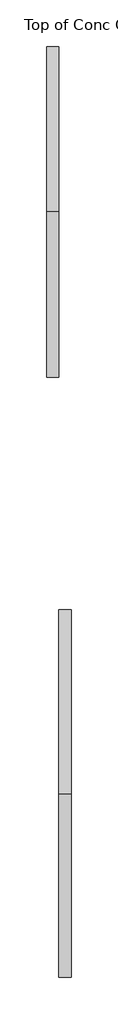
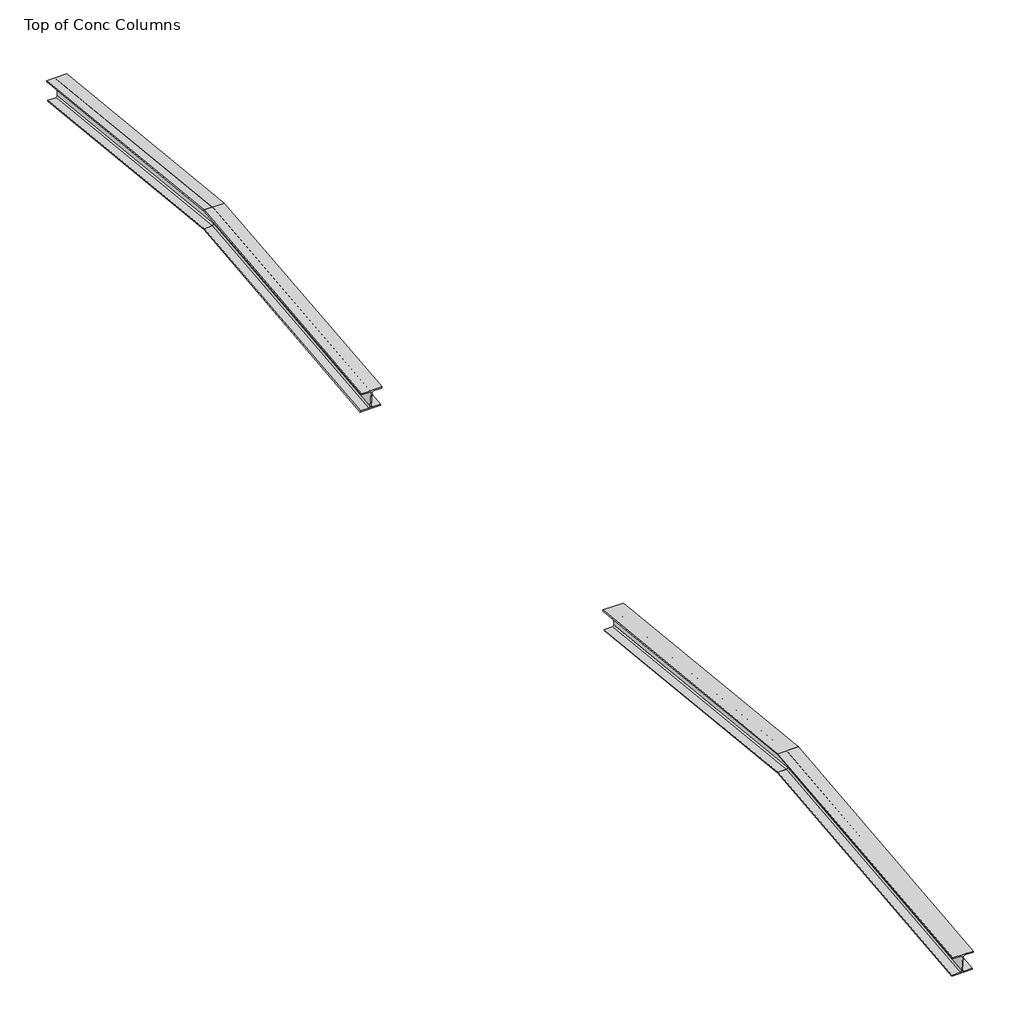
# One storey: 4 beams.
"""IFC4 building model written with IfcOpenShell, lengths in millimetres."""

from ifc_helpers import new_model, si_unit, frame, origin, place, context, project, spatial, polyline, circle_curve, ellipse_curve, element, save
from ifc_brep_helpers import plane_surface, revolved_surface, advanced_brep

model = new_model("IFC4")

# Units and contexts
model_context = context("Model", 3, world=origin())
ifc_project = project(units=[si_unit("LENGTHUNIT", "METRE", prefix="MILLI")], contexts=[model_context])

# Site, building, storey
site = spatial("IfcSite", under=ifc_project)
building = spatial("IfcBuilding", under=site)
storey = spatial("IfcBuildingStorey", under=building, Name="Top of Conc Columns", Elevation=33782.0)

# Beams
placement = place(None, origin())
element("IfcBeam", 1, ObjectType="W-Wide Flange : W12X79", at=placement, inside=storey, context=model_context, shape_type="AdvancedBrep", body=[
    advanced_brep(
    [(-21755.4154607, 20969.2190095, 33178.8039345), (-21630.3204607, 20969.2190095, 33178.8039345), (-21607.7144607, 20971.5967656, 33201.2845375), (-21607.7144607, 20996.0422355, 33432.4053438), (-21630.3204607, 20998.4199915, 33454.8859468), (-21755.4154607, 20998.4199915, 33454.8859468), (-21755.4154607, 21000.383644, 33473.4513887), (-21448.0754607, 21000.383644, 33473.4513887), (-21448.0754607, 20998.4199915, 33454.8859468), (-21573.1704607, 20998.4199915, 33454.8859468), (-21595.7764607, 20996.0422355, 33432.4053438), (-21595.7764607, 20971.5967656, 33201.2845375), (-21573.1704607, 20969.2190095, 33178.8039345), (-21448.0754607, 20969.2190095, 33178.8039345), (-21448.0754607, 20967.255357, 33160.2384927), (-21755.4154607, 20967.255357, 33160.2384927), (-21755.4154607, 16882.4695005, 33611.0562864), (-21630.3204607, 16882.4695005, 33611.0562864), (-21607.7144607, 16882.4695005, 33633.7883829), (-21607.7144607, 16882.4695005, 33867.4947677), (-21630.3204607, 16882.4695005, 33890.2268642), (-21755.4154607, 16882.4695005, 33890.2268642), (-21755.4154607, 16882.4695005, 33909.0), (-21448.0754607, 16882.4695005, 33909.0), (-21448.0754607, 16882.4695005, 33890.2268642), (-21573.1704607, 16882.4695005, 33890.2268642), (-21595.7764607, 16882.4695005, 33867.4947677), (-21595.7764607, 16882.4695005, 33633.7883829), (-21573.1704607, 16882.4695005, 33611.0562864), (-21448.0754607, 16882.4695005, 33611.0562864), (-21448.0754607, 16882.4695005, 33592.2831506), (-21755.4154607, 16882.4695005, 33592.2831506)],
    [
        (0, 1),
        (1, 2, circle_curve(frame((-21630.3204607, 20971.5967656, 33201.2845375), z_axis=(0.0, -0.9944529335787645, 0.10518252182083104), x_axis=(1.0, 0.0, 0.0)), 22.606)),
        (2, 3),
        (3, 4, circle_curve(frame((-21630.3204607, 20996.0422355, 33432.4053438), z_axis=(0.0, -0.9944529335787645, 0.10518252182083104), x_axis=(1.0, 0.0, 0.0)), 22.606)),
        (4, 5),
        (5, 6),
        (6, 7),
        (7, 8),
        (8, 9),
        (9, 10, circle_curve(frame((-21573.1704607, 20996.0422355, 33432.4053438), z_axis=(0.0, -0.9944529335787645, 0.10518252182083104), x_axis=(1.0, 0.0, 0.0)), 22.606)),
        (10, 11),
        (11, 12, circle_curve(frame((-21573.1704607, 20971.5967656, 33201.2845375), z_axis=(0.0, -0.9944529335787645, 0.10518252182083104), x_axis=(1.0, 0.0, 0.0)), 22.606)),
        (12, 13),
        (13, 14),
        (14, 15),
        (15, 0),
        (0, 16),
        (16, 17),
        (17, 1),
        (17, 18, ellipse_curve(frame((-21630.3204607, 16882.4695005, 33633.7883829), z_axis=(0.0, -1.0, 0.0), x_axis=(0.0, 0.0, 0.9999999999999999)), 22.7320964, 22.606)),
        (18, 2),
        (18, 19),
        (19, 3),
        (19, 20, ellipse_curve(frame((-21630.3204607, 16882.4695005, 33867.4947677), z_axis=(0.0, -1.0, 0.0), x_axis=(0.0, 0.0, 0.9999999999999999)), 22.7320964, 22.606)),
        (20, 4),
        (20, 21),
        (21, 5),
        (21, 22),
        (22, 6),
        (22, 23),
        (23, 7),
        (23, 24),
        (24, 8),
        (24, 25),
        (25, 9),
        (25, 26, ellipse_curve(frame((-21573.1704607, 16882.4695005, 33867.4947677), z_axis=(0.0, -1.0, 0.0), x_axis=(0.0, 0.0, 0.9999999999999999)), 22.7320964, 22.606)),
        (26, 10),
        (26, 27),
        (27, 11),
        (27, 28, ellipse_curve(frame((-21573.1704607, 16882.4695005, 33633.7883829), z_axis=(0.0, -1.0, 0.0), x_axis=(0.0, 0.0, 0.9999999999999999)), 22.7320964, 22.606)),
        (28, 12),
        (28, 29),
        (29, 13),
        (29, 30),
        (30, 14),
        (30, 31),
        (31, 15),
        (31, 16),
    ],
    [
        plane_surface(frame((-21601.7454607, 20983.8195005, 33316.8449407), z_axis=(0.0, 0.9944529335787644, -0.10518252182083183), x_axis=(0.0, 0.10518252182083183, 0.9944529335787644))),
        plane_surface(frame((-21755.4154607, 20969.2190095, 33178.8039345), z_axis=(0.0, 0.10518252182083103, 0.9944529335787644), x_axis=(0.0, -0.9944529335787644, 0.10518252182083103))),
        revolved_surface(polyline([(-21607.7144607, 16880.091744411304, 33634.03987627958), (-21607.7144607, 20971.5967656, 33201.2845375)]), (-21630.3204607, 20971.5967656, 33201.2845375), (0.0, -0.9944529335787643, 0.10518252182083102)),
        plane_surface(frame((-21607.7144607, 20971.5967656, 33201.2845375), z_axis=(-1.0, 0.0, 0.0), x_axis=(0.0, -0.9944529335787644, 0.10518252182083103))),
        revolved_surface(polyline([(-21607.7144607, 16880.09174440577, 33867.74626112727), (-21607.7144607, 20996.0422355, 33432.4053438)]), (-21630.3204607, 20996.0422355, 33432.4053438), (0.0, -0.9944529335787643, 0.10518252182083102)),
        plane_surface(frame((-21630.3204607, 20998.4199915, 33454.8859468), z_axis=(0.0, -0.10518252182083103, -0.9944529335787644), x_axis=(0.0, -0.9944529335787644, 0.10518252182083103))),
        plane_surface(frame((-21755.4154607, 20998.4199915, 33454.8859468), z_axis=(-1.0, 0.0, 0.0), x_axis=(0.0, -0.9944529335787644, 0.10518252182083103))),
        plane_surface(frame((-21755.4154607, 21000.383644, 33473.4513887), z_axis=(0.0, 0.10518252182083103, 0.9944529335787644), x_axis=(0.0, -0.9944529335787644, 0.10518252182083103))),
        plane_surface(frame((-21448.0754607, 21000.383644, 33473.4513887), z_axis=(1.0, 0.0, 0.0), x_axis=(0.0, -0.9944529335787644, 0.10518252182083103))),
        plane_surface(frame((-21448.0754607, 20998.4199915, 33454.8859468), z_axis=(0.0, -0.10518252182083103, -0.9944529335787644), x_axis=(0.0, -0.9944529335787644, 0.10518252182083103))),
        revolved_surface(polyline([(-21550.5644607, 16880.09174440577, 33867.74626112727), (-21550.5644607, 20996.0422355, 33432.4053438)]), (-21573.1704607, 20996.0422355, 33432.4053438), (0.0, -0.9944529335787643, 0.10518252182083102)),
        plane_surface(frame((-21595.7764607, 20996.0422355, 33432.4053438), z_axis=(1.0, 0.0, 0.0), x_axis=(0.0, -0.9944529335787644, 0.10518252182083103))),
        revolved_surface(polyline([(-21550.5644607, 16880.091744411304, 33634.03987627958), (-21550.5644607, 20971.5967656, 33201.2845375)]), (-21573.1704607, 20971.5967656, 33201.2845375), (0.0, -0.9944529335787643, 0.10518252182083102)),
        plane_surface(frame((-21573.1704607, 20969.2190095, 33178.8039345), z_axis=(0.0, 0.10518252182083103, 0.9944529335787644), x_axis=(0.0, -0.9944529335787644, 0.10518252182083103))),
        plane_surface(frame((-21448.0754607, 20969.2190095, 33178.8039345), z_axis=(1.0, 0.0, 0.0), x_axis=(0.0, -0.9944529335787644, 0.10518252182083103))),
        plane_surface(frame((-21448.0754607, 20967.255357, 33160.2384927), z_axis=(0.0, -0.10518252182083103, -0.9944529335787644), x_axis=(0.0, -0.9944529335787644, 0.10518252182083103))),
        plane_surface(frame((-21755.4154607, 20967.255357, 33160.2384927), z_axis=(-1.0, 0.0, 0.0), x_axis=(0.0, -0.9944529335787644, 0.10518252182083103))),
        plane_surface(frame((-21601.7454607, 16882.4695005, 33592.2831506), z_axis=(0.0, -1.0, 0.0), x_axis=(0.0, 0.0, 1.0))),
    ],
    [
        (0, [[1, 2, 3, 4, 5, 6, 7, 8, 9, 10, 11, 12, 13, 14, 15, 16]]),
        (1, [[-1, 17, 18, 19]]),
        (2, [[-2, -19, 20, 21]]),
        (3, [[-3, -21, 22, 23]]),
        (4, [[-4, -23, 24, 25]]),
        (5, [[-5, -25, 26, 27]]),
        (6, [[-6, -27, 28, 29]]),
        (7, [[-7, -29, 30, 31]]),
        (8, [[-8, -31, 32, 33]]),
        (9, [[-9, -33, 34, 35]]),
        (10, [[-10, -35, 36, 37]]),
        (11, [[-11, -37, 38, 39]]),
        (12, [[-12, -39, 40, 41]]),
        (13, [[-13, -41, 42, 43]]),
        (14, [[-14, -43, 44, 45]]),
        (15, [[-15, -45, 46, 47]]),
        (16, [[-16, -47, 48, -17]]),
        (17, [[-48, -46, -44, -42, -40, -38, -36, -34, -32, -30, -28, -26, -24, -22, -20, -18]]),
    ],
),
])
element("IfcBeam", 2, ObjectType="W-Wide Flange : W12X79", at=placement, inside=storey, context=model_context, shape_type="AdvancedBrep", body=[
    advanced_brep(
    [(-21755.4154607, 12795.7199915, 33178.8039345), (-21755.4154607, 12797.683644, 33160.2384927), (-21448.0754607, 12797.683644, 33160.2384927), (-21448.0754607, 12795.7199915, 33178.8039345), (-21573.1704607, 12795.7199915, 33178.8039345), (-21595.7764607, 12793.3422355, 33201.2845375), (-21595.7764607, 12768.8967656, 33432.4053438), (-21573.1704607, 12766.5190095, 33454.8859468), (-21448.0754607, 12766.5190095, 33454.8859468), (-21448.0754607, 12764.555357, 33473.4513887), (-21755.4154607, 12764.555357, 33473.4513887), (-21755.4154607, 12766.5190095, 33454.8859468), (-21630.3204607, 12766.5190095, 33454.8859468), (-21607.7144607, 12768.8967656, 33432.4053438), (-21607.7144607, 12793.3422355, 33201.2845375), (-21630.3204607, 12795.7199915, 33178.8039345), (-21630.3204607, 16882.4695005, 33611.0562864), (-21755.4154607, 16882.4695005, 33611.0562864), (-21607.7144607, 16882.4695005, 33633.7883829), (-21607.7144607, 16882.4695005, 33867.4947677), (-21630.3204607, 16882.4695005, 33890.2268642), (-21755.4154607, 16882.4695005, 33890.2268642), (-21755.4154607, 16882.4695005, 33909.0), (-21448.0754607, 16882.4695005, 33909.0), (-21448.0754607, 16882.4695005, 33890.2268642), (-21573.1704607, 16882.4695005, 33890.2268642), (-21595.7764607, 16882.4695005, 33867.4947677), (-21595.7764607, 16882.4695005, 33633.7883829), (-21573.1704607, 16882.4695005, 33611.0562864), (-21448.0754607, 16882.4695005, 33611.0562864), (-21448.0754607, 16882.4695005, 33592.2831506), (-21755.4154607, 16882.4695005, 33592.2831506)],
    [
        (0, 1),
        (1, 2),
        (2, 3),
        (3, 4),
        (4, 5, circle_curve(frame((-21573.1704607, 12793.3422355, 33201.2845375), z_axis=(0.0, 0.9944529335787644, 0.10518252182083103), x_axis=(1.0, 0.0, 0.0)), 22.606)),
        (5, 6),
        (6, 7, circle_curve(frame((-21573.1704607, 12768.8967656, 33432.4053438), z_axis=(0.0, 0.9944529335787644, 0.10518252182083103), x_axis=(1.0, 0.0, 0.0)), 22.606)),
        (7, 8),
        (8, 9),
        (9, 10),
        (10, 11),
        (11, 12),
        (12, 13, circle_curve(frame((-21630.3204607, 12768.8967656, 33432.4053438), z_axis=(0.0, 0.9944529335787644, 0.10518252182083103), x_axis=(1.0, 0.0, 0.0)), 22.606)),
        (13, 14),
        (14, 15, circle_curve(frame((-21630.3204607, 12793.3422355, 33201.2845375), z_axis=(0.0, 0.9944529335787644, 0.10518252182083103), x_axis=(1.0, 0.0, 0.0)), 22.606)),
        (15, 0),
        (15, 16),
        (16, 17),
        (17, 0),
        (14, 18),
        (18, 16, ellipse_curve(frame((-21630.3204607, 16882.4695005, 33633.7883829), z_axis=(0.0, 1.0, 0.0), x_axis=(0.0, 0.0, 1.0)), 22.7320964, 22.606)),
        (13, 19),
        (19, 18),
        (12, 20),
        (20, 19, ellipse_curve(frame((-21630.3204607, 16882.4695005, 33867.4947677), z_axis=(0.0, 1.0, 0.0), x_axis=(0.0, 0.0, 1.0)), 22.7320964, 22.606)),
        (11, 21),
        (21, 20),
        (10, 22),
        (22, 21),
        (9, 23),
        (23, 22),
        (8, 24),
        (24, 23),
        (7, 25),
        (25, 24),
        (6, 26),
        (26, 25, ellipse_curve(frame((-21573.1704607, 16882.4695005, 33867.4947677), z_axis=(0.0, 1.0, 0.0), x_axis=(0.0, 0.0, 1.0)), 22.7320964, 22.606)),
        (5, 27),
        (27, 26),
        (4, 28),
        (28, 27, ellipse_curve(frame((-21573.1704607, 16882.4695005, 33633.7883829), z_axis=(0.0, 1.0, 0.0), x_axis=(0.0, 0.0, 1.0)), 22.7320964, 22.606)),
        (3, 29),
        (29, 28),
        (2, 30),
        (30, 29),
        (1, 31),
        (31, 30),
        (17, 31),
    ],
    [
        plane_surface(frame((-21601.7454607, 12781.1195005, 33316.8449407), z_axis=(0.0, -0.9944529335787644, -0.10518252182083185), x_axis=(0.0, -0.10518252182083185, 0.9944529335787644))),
        plane_surface(frame((-21755.4154607, 12795.7199915, 33178.8039345), z_axis=(0.0, -0.10518252182083103, 0.9944529335787644), x_axis=(0.0, 0.9944529335787644, 0.10518252182083103))),
        revolved_surface(polyline([(-21607.7144607, 16884.847256589805, 33634.03987626912), (-21607.7144607, 12793.342235414419, 33201.28453749095)]), (-21630.3204607, 12793.3422355, 33201.2845375), (0.0, 0.9944529335787644, 0.10518252182083103)),
        plane_surface(frame((-21607.7144607, 12793.3422355, 33201.2845375), z_axis=(-1.0, 0.0, 0.0), x_axis=(0.0, 0.9944529335787644, 0.10518252182083103))),
        revolved_surface(polyline([(-21607.7144607, 16884.847256595338, 33867.746261116816), (-21607.7144607, 12768.896765586687, 33432.405343798586)]), (-21630.3204607, 12768.8967656, 33432.4053438), (0.0, 0.9944529335787644, 0.10518252182083103)),
        plane_surface(frame((-21630.3204607, 12766.5190095, 33454.8859468), z_axis=(0.0, 0.10518252182083103, -0.9944529335787644), x_axis=(0.0, 0.9944529335787644, 0.10518252182083103))),
        plane_surface(frame((-21755.4154607, 12766.5190095, 33454.8859468), z_axis=(-1.0, 0.0, 0.0), x_axis=(0.0, 0.9944529335787644, 0.10518252182083103))),
        plane_surface(frame((-21755.4154607, 12764.555357, 33473.4513887), z_axis=(0.0, -0.10518252182083103, 0.9944529335787644), x_axis=(0.0, 0.9944529335787644, 0.10518252182083103))),
        plane_surface(frame((-21448.0754607, 12764.555357, 33473.4513887), z_axis=(1.0, 0.0, 0.0), x_axis=(0.0, 0.9944529335787644, 0.10518252182083103))),
        plane_surface(frame((-21448.0754607, 12766.5190095, 33454.8859468), z_axis=(0.0, 0.10518252182083103, -0.9944529335787644), x_axis=(0.0, 0.9944529335787644, 0.10518252182083103))),
        revolved_surface(polyline([(-21550.5644607, 16884.847256595338, 33867.746261116816), (-21550.5644607, 12768.896765586687, 33432.405343798586)]), (-21573.1704607, 12768.8967656, 33432.4053438), (0.0, 0.9944529335787644, 0.10518252182083103)),
        plane_surface(frame((-21595.7764607, 12768.8967656, 33432.4053438), z_axis=(1.0, 0.0, 0.0), x_axis=(0.0, 0.9944529335787644, 0.10518252182083103))),
        revolved_surface(polyline([(-21550.5644607, 16884.847256589805, 33634.03987626912), (-21550.5644607, 12793.342235414419, 33201.28453749095)]), (-21573.1704607, 12793.3422355, 33201.2845375), (0.0, 0.9944529335787644, 0.10518252182083103)),
        plane_surface(frame((-21573.1704607, 12795.7199915, 33178.8039345), z_axis=(0.0, -0.10518252182083103, 0.9944529335787644), x_axis=(0.0, 0.9944529335787644, 0.10518252182083103))),
        plane_surface(frame((-21448.0754607, 12795.7199915, 33178.8039345), z_axis=(1.0, 0.0, 0.0), x_axis=(0.0, 0.9944529335787644, 0.10518252182083103))),
        plane_surface(frame((-21448.0754607, 12797.683644, 33160.2384927), z_axis=(0.0, 0.10518252182083103, -0.9944529335787644), x_axis=(0.0, 0.9944529335787644, 0.10518252182083103))),
        plane_surface(frame((-21755.4154607, 12797.683644, 33160.2384927), z_axis=(-1.0, 0.0, 0.0), x_axis=(0.0, 0.9944529335787644, 0.10518252182083103))),
        plane_surface(frame((-21601.7454607, 16882.4695005, 33592.2831506), z_axis=(0.0, 1.0, 0.0), x_axis=(0.0, 0.0, -1.0))),
    ],
    [
        (0, [[1, 2, 3, 4, 5, 6, 7, 8, 9, 10, 11, 12, 13, 14, 15, 16]]),
        (1, [[17, 18, 19, -16]]),
        (2, [[20, 21, -17, -15]]),
        (3, [[22, 23, -20, -14]]),
        (4, [[24, 25, -22, -13]]),
        (5, [[26, 27, -24, -12]]),
        (6, [[28, 29, -26, -11]]),
        (7, [[30, 31, -28, -10]]),
        (8, [[32, 33, -30, -9]]),
        (9, [[34, 35, -32, -8]]),
        (10, [[36, 37, -34, -7]]),
        (11, [[38, 39, -36, -6]]),
        (12, [[40, 41, -38, -5]]),
        (13, [[42, 43, -40, -4]]),
        (14, [[44, 45, -42, -3]]),
        (15, [[46, 47, -44, -2]]),
        (16, [[-19, 48, -46, -1]]),
        (17, [[-18, -21, -23, -25, -27, -29, -31, -33, -35, -37, -39, -41, -43, -45, -47, -48]]),
    ],
),
])
element("IfcBeam", 3, ObjectType="W-Wide Flange : W12X79", at=placement, inside=storey, context=model_context, shape_type="AdvancedBrep", body=[
    advanced_brep(
    [(-21450.6154607, 6948.4190095, 33130.4462422), (-21325.5204607, 6948.4190095, 33130.4462422), (-21302.9144607, 6950.7967656, 33152.9268452), (-21302.9144607, 6975.2422355, 33384.0476515), (-21325.5204607, 6977.6199915, 33406.5282545), (-21450.6154607, 6977.6199915, 33406.5282545), (-21450.6154607, 6979.583644, 33425.0936964), (-21143.2754607, 6979.583644, 33425.0936964), (-21143.2754607, 6977.6199915, 33406.5282545), (-21268.3704607, 6977.6199915, 33406.5282545), (-21290.9764607, 6975.2422355, 33384.0476515), (-21290.9764607, 6950.7967656, 33152.9268452), (-21268.3704607, 6948.4190095, 33130.4462422), (-21143.2754607, 6948.4190095, 33130.4462422), (-21143.2754607, 6946.455357, 33111.8808004), (-21450.6154607, 6946.455357, 33111.8808004), (-21450.6154607, 2404.4695005, 33611.0562864), (-21325.5204607, 2404.4695005, 33611.0562864), (-21302.9144607, 2404.4695005, 33633.7883829), (-21302.9144607, 2404.4695005, 33867.4947677), (-21325.5204607, 2404.4695005, 33890.2268642), (-21450.6154607, 2404.4695005, 33890.2268642), (-21450.6154607, 2404.4695005, 33909.0), (-21143.2754607, 2404.4695005, 33909.0), (-21143.2754607, 2404.4695005, 33890.2268642), (-21268.3704607, 2404.4695005, 33890.2268642), (-21290.9764607, 2404.4695005, 33867.4947677), (-21290.9764607, 2404.4695005, 33633.7883829), (-21268.3704607, 2404.4695005, 33611.0562864), (-21143.2754607, 2404.4695005, 33611.0562864), (-21143.2754607, 2404.4695005, 33592.2831506), (-21450.6154607, 2404.4695005, 33592.2831506)],
    [
        (0, 1),
        (1, 2, circle_curve(frame((-21325.5204607, 6950.7967656, 33152.9268452), z_axis=(0.0, -0.9944529335787645, 0.10518252182083104), x_axis=(0.9999999999999999, 0.0, 0.0)), 22.606)),
        (2, 3),
        (3, 4, circle_curve(frame((-21325.5204607, 6975.2422355, 33384.0476515), z_axis=(0.0, -0.9944529335787645, 0.10518252182083104), x_axis=(0.0, 0.10518252182083125, 0.9944529335787644)), 22.606)),
        (4, 5),
        (5, 6),
        (6, 7),
        (7, 8),
        (8, 9),
        (9, 10, circle_curve(frame((-21268.3704607, 6975.2422355, 33384.0476515), z_axis=(0.0, -0.9944529335787645, 0.10518252182083104), x_axis=(-0.9999999999999999, 0.0, 0.0)), 22.606)),
        (10, 11),
        (11, 12, circle_curve(frame((-21268.3704607, 6950.7967656, 33152.9268452), z_axis=(0.0, -0.9944529335787645, 0.10518252182083104), x_axis=(0.0, -0.10518252182083125, -0.9944529335787644)), 22.606)),
        (12, 13),
        (13, 14),
        (14, 15),
        (15, 0),
        (0, 16),
        (16, 17),
        (17, 1),
        (17, 18, ellipse_curve(frame((-21325.5204607, 2404.4695005, 33633.7883829), z_axis=(0.0, -1.0, 0.0), x_axis=(0.0, 0.0, 0.9999999999999999)), 22.7320964, 22.606)),
        (18, 2),
        (18, 19),
        (19, 3),
        (19, 20, ellipse_curve(frame((-21325.5204607, 2404.4695005, 33867.4947677), z_axis=(0.0, -1.0, 0.0), x_axis=(0.0, 0.0, 0.9999999999999999)), 22.7320964, 22.606)),
        (20, 4),
        (20, 21),
        (21, 5),
        (21, 22),
        (22, 6),
        (22, 23),
        (23, 7),
        (23, 24),
        (24, 8),
        (24, 25),
        (25, 9),
        (25, 26, ellipse_curve(frame((-21268.3704607, 2404.4695005, 33867.4947677), z_axis=(0.0, -1.0, 0.0), x_axis=(0.0, 0.0, 0.9999999999999999)), 22.7320964, 22.606)),
        (26, 10),
        (26, 27),
        (27, 11),
        (27, 28, ellipse_curve(frame((-21268.3704607, 2404.4695005, 33633.7883829), z_axis=(0.0, -1.0, 0.0), x_axis=(0.0, 0.0, 0.9999999999999999)), 22.7320964, 22.606)),
        (28, 12),
        (28, 29),
        (29, 13),
        (29, 30),
        (30, 14),
        (30, 31),
        (31, 15),
        (31, 16),
    ],
    [
        plane_surface(frame((-21296.9454607, 6963.0195005, 33268.4872484), z_axis=(0.0, 0.9944529335787644, -0.10518252182083125), x_axis=(0.0, 0.10518252182083125, 0.9944529335787644))),
        plane_surface(frame((-21388.0679607, 6948.4190095, 33130.4462422), z_axis=(0.0, 0.10518252182083103, 0.9944529335787644), x_axis=(1.0, 0.0, 0.0))),
        revolved_surface(polyline([(-21302.9144607, 2402.091744412107, 33634.039876287185), (-21302.9144607, 6950.7967656, 33152.9268452)]), (-21325.5204607, 6950.7967656, 33152.9268452), (0.0, -0.9944529335787643, 0.10518252182083102)),
        plane_surface(frame((-21302.9144607, 6963.0195005, 33268.4872484), z_axis=(-1.0, 0.0, 0.0), x_axis=(0.0, 0.10518252182083125, 0.9944529335787644))),
        revolved_surface(polyline([(-21325.5204607, 2404.4695004948553, 33890.226864151366), (-21325.5204607, 6977.619991588282, 33406.52825451648)]), (-21325.5204607, 6975.2422355, 33384.0476515), (0.0, -0.9944529335787643, 0.10518252182083102)),
        plane_surface(frame((-21388.0679607, 6977.6199915, 33406.5282545), z_axis=(0.0, -0.10518252182083103, -0.9944529335787644), x_axis=(-1.0, 0.0, 0.0))),
        plane_surface(frame((-21450.6154607, 6978.6018178, 33415.8109754), z_axis=(-1.0, 0.0, 0.0), x_axis=(0.0, 0.10518252182083125, 0.9944529335787644))),
        plane_surface(frame((-21296.9454607, 6979.583644, 33425.0936964), z_axis=(0.0, 0.10518252182083103, 0.9944529335787644), x_axis=(1.0, 0.0, 0.0))),
        plane_surface(frame((-21143.2754607, 6978.6018178, 33415.8109754), z_axis=(1.0, 0.0, 0.0), x_axis=(0.0, -0.10518252182083125, -0.9944529335787644))),
        plane_surface(frame((-21205.8229607, 6977.6199915, 33406.5282545), z_axis=(0.0, -0.10518252182083103, -0.9944529335787644), x_axis=(-1.0, 0.0, 0.0))),
        revolved_surface(polyline([(-21290.9764607, 2402.0917444065735, 33867.74626113488), (-21290.9764607, 6975.2422355, 33384.0476515)]), (-21268.3704607, 6975.2422355, 33384.0476515), (0.0, -0.9944529335787643, 0.10518252182083102)),
        plane_surface(frame((-21290.9764607, 6963.0195005, 33268.4872484), z_axis=(1.0, 0.0, 0.0), x_axis=(0.0, -0.10518252182083125, -0.9944529335787644))),
        revolved_surface(polyline([(-21268.3704607, 2399.713988323825, 33611.5592732707), (-21268.3704607, 6948.419009511718, 33130.44624218352)]), (-21268.3704607, 6950.7967656, 33152.9268452), (0.0, -0.9944529335787643, 0.10518252182083102)),
        plane_surface(frame((-21205.8229607, 6948.4190095, 33130.4462422), z_axis=(0.0, 0.10518252182083103, 0.9944529335787644), x_axis=(1.0, 0.0, 0.0))),
        plane_surface(frame((-21143.2754607, 6947.4371832, 33121.1635213), z_axis=(1.0, 0.0, 0.0), x_axis=(0.0, -0.10518252182083125, -0.9944529335787644))),
        plane_surface(frame((-21296.9454607, 6946.455357, 33111.8808004), z_axis=(0.0, -0.10518252182083103, -0.9944529335787644), x_axis=(-1.0, 0.0, 0.0))),
        plane_surface(frame((-21450.6154607, 6947.4371832, 33121.1635213), z_axis=(-1.0, 0.0, 0.0), x_axis=(0.0, 0.10518252182083125, 0.9944529335787644))),
        plane_surface(frame((-21296.9454607, 2404.4695005, 33592.2831506), z_axis=(0.0, -1.0, 0.0), x_axis=(0.0, 0.0, 1.0))),
    ],
    [
        (0, [[1, 2, 3, 4, 5, 6, 7, 8, 9, 10, 11, 12, 13, 14, 15, 16]]),
        (1, [[-1, 17, 18, 19]]),
        (2, [[-2, -19, 20, 21]]),
        (3, [[-3, -21, 22, 23]]),
        (4, [[-4, -23, 24, 25]]),
        (5, [[-5, -25, 26, 27]]),
        (6, [[-6, -27, 28, 29]]),
        (7, [[-7, -29, 30, 31]]),
        (8, [[-8, -31, 32, 33]]),
        (9, [[-9, -33, 34, 35]]),
        (10, [[-10, -35, 36, 37]]),
        (11, [[-11, -37, 38, 39]]),
        (12, [[-12, -39, 40, 41]]),
        (13, [[-13, -41, 42, 43]]),
        (14, [[-14, -43, 44, 45]]),
        (15, [[-15, -45, 46, 47]]),
        (16, [[-16, -47, 48, -17]]),
        (17, [[-48, -46, -44, -42, -40, -38, -36, -34, -32, -30, -28, -26, -24, -22, -20, -18]]),
    ],
),
])
element("IfcBeam", 4, ObjectType="W-Wide Flange : W12X79", at=placement, inside=storey, context=model_context, shape_type="AdvancedBrep", body=[
    advanced_brep(
    [(-21450.6154607, -2139.4800085, 33130.4462422), (-21450.6154607, -2137.516356, 33111.8808004), (-21143.2754607, -2137.516356, 33111.8808004), (-21143.2754607, -2139.4800085, 33130.4462422), (-21268.3704607, -2139.4800085, 33130.4462422), (-21290.9764607, -2141.8577645, 33152.9268452), (-21290.9764607, -2166.3032344, 33384.0476515), (-21268.3704607, -2168.6809905, 33406.5282545), (-21143.2754607, -2168.6809905, 33406.5282545), (-21143.2754607, -2170.644643, 33425.0936964), (-21450.6154607, -2170.644643, 33425.0936964), (-21450.6154607, -2168.6809905, 33406.5282545), (-21325.5204607, -2168.6809905, 33406.5282545), (-21302.9144607, -2166.3032344, 33384.0476515), (-21302.9144607, -2141.8577645, 33152.9268452), (-21325.5204607, -2139.4800085, 33130.4462422), (-21325.5204607, 2404.4695005, 33611.0562864), (-21450.6154607, 2404.4695005, 33611.0562864), (-21302.9144607, 2404.4695005, 33633.7883829), (-21302.9144607, 2404.4695005, 33867.4947677), (-21325.5204607, 2404.4695005, 33890.2268642), (-21450.6154607, 2404.4695005, 33890.2268642), (-21450.6154607, 2404.4695005, 33909.0), (-21143.2754607, 2404.4695005, 33909.0), (-21143.2754607, 2404.4695005, 33890.2268642), (-21268.3704607, 2404.4695005, 33890.2268642), (-21290.9764607, 2404.4695005, 33867.4947677), (-21290.9764607, 2404.4695005, 33633.7883829), (-21268.3704607, 2404.4695005, 33611.0562864), (-21143.2754607, 2404.4695005, 33611.0562864), (-21143.2754607, 2404.4695005, 33592.2831506), (-21450.6154607, 2404.4695005, 33592.2831506)],
    [
        (0, 1),
        (1, 2),
        (2, 3),
        (3, 4),
        (4, 5, circle_curve(frame((-21268.3704607, -2141.8577645, 33152.9268452), z_axis=(0.0, 0.9944529335787644, 0.10518252182083103), x_axis=(0.0, 0.1051825218208312, -0.9944529335787644)), 22.606)),
        (5, 6),
        (6, 7, circle_curve(frame((-21268.3704607, -2166.3032344, 33384.0476515), z_axis=(0.0, 0.9944529335787644, 0.10518252182083103), x_axis=(-1.0, 0.0, 0.0)), 22.606)),
        (7, 8),
        (8, 9),
        (9, 10),
        (10, 11),
        (11, 12),
        (12, 13, circle_curve(frame((-21325.5204607, -2166.3032344, 33384.0476515), z_axis=(0.0, 0.9944529335787644, 0.10518252182083103), x_axis=(0.0, -0.1051825218208312, 0.9944529335787644)), 22.606)),
        (13, 14),
        (14, 15, circle_curve(frame((-21325.5204607, -2141.8577645, 33152.9268452), z_axis=(0.0, 0.9944529335787644, 0.10518252182083103), x_axis=(1.0, 0.0, 0.0)), 22.606)),
        (15, 0),
        (15, 16),
        (16, 17),
        (17, 0),
        (14, 18),
        (18, 16, ellipse_curve(frame((-21325.5204607, 2404.4695005, 33633.7883829), z_axis=(0.0, 1.0, 0.0), x_axis=(0.0, 0.0, 1.0)), 22.7320964, 22.606)),
        (13, 19),
        (19, 18),
        (12, 20),
        (20, 19, ellipse_curve(frame((-21325.5204607, 2404.4695005, 33867.4947677), z_axis=(0.0, 1.0, 0.0), x_axis=(0.0, 0.0, 1.0)), 22.7320964, 22.606)),
        (11, 21),
        (21, 20),
        (10, 22),
        (22, 21),
        (9, 23),
        (23, 22),
        (8, 24),
        (24, 23),
        (7, 25),
        (25, 24),
        (6, 26),
        (26, 25, ellipse_curve(frame((-21268.3704607, 2404.4695005, 33867.4947677), z_axis=(0.0, 1.0, 0.0), x_axis=(0.0, 0.0, 1.0)), 22.7320964, 22.606)),
        (5, 27),
        (27, 26),
        (4, 28),
        (28, 27, ellipse_curve(frame((-21268.3704607, 2404.4695005, 33633.7883829), z_axis=(0.0, 1.0, 0.0), x_axis=(0.0, 0.0, 1.0)), 22.7320964, 22.606)),
        (3, 29),
        (29, 28),
        (2, 30),
        (30, 29),
        (1, 31),
        (31, 30),
        (17, 31),
    ],
    [
        plane_surface(frame((-21296.9454607, -2154.0804995, 33268.4872484), z_axis=(0.0, -0.9944529335787644, -0.1051825218208312), x_axis=(0.0, -0.1051825218208312, 0.9944529335787644))),
        plane_surface(frame((-21388.0679607, -2139.4800085, 33130.4462422), z_axis=(0.0, -0.10518252182083103, 0.9944529335787644), x_axis=(1.0, 0.0, 0.0))),
        revolved_surface(polyline([(-21302.9144607, 2406.847256589, 33634.03987627672), (-21302.9144607, -2141.8577645855817, 33152.92684519095)]), (-21325.5204607, -2141.8577645, 33152.9268452), (0.0, 0.9944529335787644, 0.10518252182083103)),
        plane_surface(frame((-21302.9144607, -2154.0804995, 33268.4872484), z_axis=(-1.0, 0.0, 0.0), x_axis=(0.0, -0.1051825218208312, 0.9944529335787644))),
        revolved_surface(polyline([(-21325.5204607, 2404.469500506251, 33890.2268641409), (-21325.5204607, -2168.680990501594, 33406.52825451507)]), (-21325.5204607, -2166.3032344, 33384.0476515), (0.0, 0.9944529335787644, 0.10518252182083103)),
        plane_surface(frame((-21388.0679607, -2168.6809905, 33406.5282545), z_axis=(0.0, 0.10518252182083103, -0.9944529335787644), x_axis=(-1.0, 0.0, 0.0))),
        plane_surface(frame((-21450.6154607, -2169.6628168, 33415.8109754), z_axis=(-1.0, 0.0, 0.0), x_axis=(0.0, -0.1051825218208312, 0.9944529335787644))),
        plane_surface(frame((-21296.9454607, -2170.644643, 33425.0936964), z_axis=(0.0, -0.10518252182083103, 0.9944529335787644), x_axis=(1.0, 0.0, 0.0))),
        plane_surface(frame((-21143.2754607, -2169.6628168, 33415.8109754), z_axis=(1.0, 0.0, 0.0), x_axis=(0.0, 0.1051825218208312, -0.9944529335787644))),
        plane_surface(frame((-21205.8229607, -2168.6809905, 33406.5282545), z_axis=(0.0, 0.10518252182083103, -0.9944529335787644), x_axis=(-1.0, 0.0, 0.0))),
        revolved_surface(polyline([(-21290.9764607, 2406.8472565945326, 33867.74626112442), (-21290.9764607, -2166.303234413312, 33384.047651498586)]), (-21268.3704607, -2166.3032344, 33384.0476515), (0.0, 0.9944529335787644, 0.10518252182083103)),
        plane_surface(frame((-21290.9764607, -2154.0804995, 33268.4872484), z_axis=(1.0, 0.0, 0.0), x_axis=(0.0, 0.1051825218208312, -0.9944529335787644))),
        revolved_surface(polyline([(-21268.3704607, 2409.225012677282, 33611.55927326024), (-21268.3704607, -2139.4800084973, 33130.44624217447)]), (-21268.3704607, -2141.8577645, 33152.9268452), (0.0, 0.9944529335787644, 0.10518252182083103)),
        plane_surface(frame((-21205.8229607, -2139.4800085, 33130.4462422), z_axis=(0.0, -0.10518252182083103, 0.9944529335787644), x_axis=(1.0, 0.0, 0.0))),
        plane_surface(frame((-21143.2754607, -2138.4981822, 33121.1635213), z_axis=(1.0, 0.0, 0.0), x_axis=(0.0, 0.1051825218208312, -0.9944529335787644))),
        plane_surface(frame((-21296.9454607, -2137.516356, 33111.8808004), z_axis=(0.0, 0.10518252182083103, -0.9944529335787644), x_axis=(-1.0, 0.0, 0.0))),
        plane_surface(frame((-21450.6154607, -2138.4981822, 33121.1635213), z_axis=(-1.0, 0.0, 0.0), x_axis=(0.0, -0.1051825218208312, 0.9944529335787644))),
        plane_surface(frame((-21296.9454607, 2404.4695005, 33592.2831506), z_axis=(0.0, 1.0, 0.0), x_axis=(0.0, 0.0, -1.0))),
    ],
    [
        (0, [[1, 2, 3, 4, 5, 6, 7, 8, 9, 10, 11, 12, 13, 14, 15, 16]]),
        (1, [[17, 18, 19, -16]]),
        (2, [[20, 21, -17, -15]]),
        (3, [[22, 23, -20, -14]]),
        (4, [[24, 25, -22, -13]]),
        (5, [[26, 27, -24, -12]]),
        (6, [[28, 29, -26, -11]]),
        (7, [[30, 31, -28, -10]]),
        (8, [[32, 33, -30, -9]]),
        (9, [[34, 35, -32, -8]]),
        (10, [[36, 37, -34, -7]]),
        (11, [[38, 39, -36, -6]]),
        (12, [[40, 41, -38, -5]]),
        (13, [[42, 43, -40, -4]]),
        (14, [[44, 45, -42, -3]]),
        (15, [[46, 47, -44, -2]]),
        (16, [[-19, 48, -46, -1]]),
        (17, [[-18, -21, -23, -25, -27, -29, -31, -33, -35, -37, -39, -41, -43, -45, -47, -48]]),
    ],
),
])

save(model, "model.ifc")

# Revit data of these elements
# Type "W-Wide Flange : W12X79"
#   Assembly Code = "B10"
#   W = 79
#   Length [instance default] = 1524 mm
#   bf = 307.34 mm
#   d = 314.96 mm
#   k = 41.275 mm
#   k2 = 22.606 mm
#   tf = 18.669 mm
#   tw = 11.938 mm
#   A = 0.0149677 m²
#   Structural Material [instance default] = Steel ASTM A992
# Element 1 (IfcBeam, "W-Wide Flange : W12X79")
#   RM User Number = 149
#   RM Unique Id = 936
#   RS Unique Id = 362611
#   Structural Material = Aluminum, Anodized Red
#   Phase Created = New Construction
#   Materials on its faces: "Aluminum, Anodized Red"
# Element 2 (IfcBeam, "W-Wide Flange : W12X79")
#   RM User Number = 150
#   RM Unique Id = 937
#   RS Unique Id = 362613
#   Structural Material = Aluminum, Anodized Red
#   Phase Created = New Construction
#   Materials on its faces: "Aluminum, Anodized Red"
# Element 3 (IfcBeam, "W-Wide Flange : W12X79")
#   RM User Number = 169
#   RM Unique Id = 956
#   RS Unique Id = 370359
#   Structural Material = Aluminum, Anodized Red
#   Phase Created = New Construction
#   Materials on its faces: "Aluminum, Anodized Red"
# Element 4 (IfcBeam, "W-Wide Flange : W12X79")
#   RM User Number = 170
#   RM Unique Id = 957
#   RS Unique Id = 370361
#   Structural Material = Aluminum, Anodized Red
#   Phase Created = New Construction
#   Materials on its faces: "Aluminum, Anodized Red"
# Materials
#   "Steel ASTM A992": class "Metal", colour RGB 128 0 0, transparency 0, Description = "Structural steel 50ksi", Cost = 0
#   "Aluminum, Anodized Red": class "Metal", colour RGB 120 120 120, transparency 0, Description = "Anodized aluminum, red", Cost = 0
